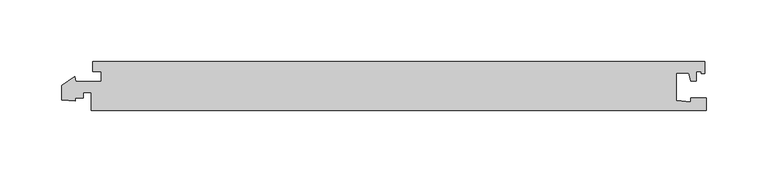
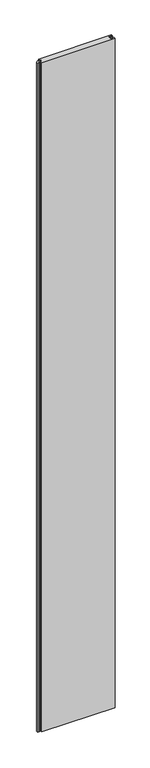
"""IFC4 building model written with IfcOpenShell, lengths in millimetres: proxy geometry, Generic Models 5:Generic Models 5:321804:Generic Models 5:321804 : Generic Models 5:Generic Models 5:321804:26 : Generic Models 5:Generic Models 5:321804:Generic Models 5:321804 : Generic Models 5:Generic Models 5:321804:300761."""

import ifcopenshell
import ifcopenshell.guid

model = None  # the IFC model being written
_history = None  # IfcOwnerHistory: only IFC2X3 demands one
_inside = {}  # id of a spatial element -> (the spatial element, [elements in it])
_under = {}  # id of a project, library or spatial element -> (it, [spatial elements below it])
_declared = {}  # id of a project -> (the project, [libraries it declares])
_typed = {}  # id of a type object -> (the type object, [elements of that type])
_made_of = {}  # id of a material, layer set ... -> (it, [elements and type objects made of it])


def new_model(schema):
    """Start an empty IFC model of exactly this schema.

    Asked for "IFC4X3", IfcOpenShell would pick the latest addendum, in which some entities
    have other attributes; the version numbers below select the first issue.
    IFC2X3 requires an IfcOwnerHistory on every rooted entity: one is made here for all.
    """
    global model, _history
    if schema == "IFC4X3":
        model = ifcopenshell.file(schema_version=(4, 3, 0, 0))
    else:
        model = ifcopenshell.file(schema=schema)
    _inside.clear()
    _under.clear()
    _declared.clear()
    _typed.clear()
    _made_of.clear()
    _history = None
    if model.schema == "IFC2X3":
        org = make("IfcOrganization", Name="unknown")
        user = make(
            "IfcPersonAndOrganization",
            ThePerson=make("IfcPerson", FamilyName="unknown"),
            TheOrganization=org,
        )
        app = make(
            "IfcApplication",
            ApplicationDeveloper=org,
            Version="unknown",
            ApplicationFullName="unknown",
            ApplicationIdentifier="unknown",
        )
        _history = make(
            "IfcOwnerHistory",
            OwningUser=user,
            OwningApplication=app,
            ChangeAction="ADDED",
            CreationDate=0,
        )
    return model


def make(cls, **values):
    """One entity of the class cls with the attributes given. An attribute that is None is left unset."""
    return model.create_entity(
        cls, **{name: value for name, value in values.items() if value is not None}
    )


def rooted(cls, **values):
    """An entity with a GlobalId (a new one), such as an element, a storey or a relation."""
    return make(cls, GlobalId=ifcopenshell.guid.new(), OwnerHistory=_history, **values)


def si_unit(unit_type, name, prefix=None):
    """IfcSIUnit, for example si_unit("LENGTHUNIT", "METRE", prefix="MILLI")."""
    return make("IfcSIUnit", UnitType=unit_type, Prefix=prefix, Name=name)


def assignment(units):
    """IfcUnitAssignment: the units of a project."""
    return None if units is None else make("IfcUnitAssignment", Units=units)


def point(xyz):
    """IfcCartesianPoint."""
    return None if xyz is None else make("IfcCartesianPoint", Coordinates=xyz)


def direction(xyz):
    """IfcDirection."""
    return None if xyz is None else make("IfcDirection", DirectionRatios=xyz)


def frame(location, z_axis=None, x_axis=None):
    """IfcAxis2Placement3D, a coordinate frame: its origin and axes. An axis left out is left unset."""
    return make(
        "IfcAxis2Placement3D",
        Location=point(location),
        Axis=direction(z_axis),
        RefDirection=direction(x_axis),
    )


def origin():
    """The frame at (0, 0, 0) with its axes left unset."""
    return frame((0.0, 0.0, 0.0))


def place(relative_to, where):
    """IfcLocalPlacement: puts the frame where relative to a parent placement (None: the world)."""
    return make(
        "IfcLocalPlacement", PlacementRelTo=relative_to, RelativePlacement=where
    )


def context(
    kind, dimensions, precision=None, world=None, true_north=None, identifier=None
):
    """IfcGeometricRepresentationContext, for example the 3D "Model" context."""
    return make(
        "IfcGeometricRepresentationContext",
        ContextIdentifier=identifier,
        ContextType=kind,
        CoordinateSpaceDimension=dimensions,
        Precision=precision,
        WorldCoordinateSystem=world,
        TrueNorth=true_north,
    )


def project(units=None, contexts=None):
    """IfcProject with its units and contexts."""
    return rooted(
        "IfcProject",
        Name="project",
        RepresentationContexts=contexts,
        UnitsInContext=assignment(units),
    )


def spatial(cls, under=None, at=None, **own):
    """A site, building, storey or space (cls), placed at a placement, below another one or the project."""
    s = rooted(cls, ObjectPlacement=at, **own)
    if under is not None:
        _under.setdefault(under.id(), (under, []))[1].append(s)
    return s


def polyline(points):
    """IfcPolyline through the points."""
    return make("IfcPolyline", Points=[point(p) for p in points])


def outline(outer, holes=None, kind="AREA"):
    """IfcArbitraryClosedProfileDef: a profile drawn as a closed curve; with holes, ...WithVoids."""
    if holes is None:
        return make("IfcArbitraryClosedProfileDef", ProfileType=kind, OuterCurve=outer)
    return make(
        "IfcArbitraryProfileDefWithVoids",
        ProfileType=kind,
        OuterCurve=outer,
        InnerCurves=holes,
    )


def extrude(swept, where, along, depth):
    """IfcExtrudedAreaSolid: the profile swept, set in the frame where, extruded along a direction by depth."""
    return make(
        "IfcExtrudedAreaSolid",
        SweptArea=swept,
        Position=where,
        ExtrudedDirection=direction(along),
        Depth=depth,
    )


def shape(context_of_items, identifier, shape_type, items):
    """IfcShapeRepresentation: the items that make up one representation, for example the "Body"."""
    return make(
        "IfcShapeRepresentation",
        ContextOfItems=context_of_items,
        RepresentationIdentifier=identifier,
        RepresentationType=shape_type,
        Items=items,
    )


def source(mapping_origin, context_of_items, identifier, shape_type, items):
    """IfcRepresentationMap: a shape defined once, which mapped items show again and again."""
    return make(
        "IfcRepresentationMap",
        MappingOrigin=mapping_origin,
        MappedRepresentation=shape(context_of_items, identifier, shape_type, items),
    )


def transform(
    local_origin,
    x_axis=None,
    y_axis=None,
    z_axis=None,
    scale=None,
    scale2=None,
    scale3=None,
    uniform=True,
):
    """IfcCartesianTransformationOperator3D, or its non-uniform kind. x_axis, y_axis, z_axis: its Axis1, 2, 3."""
    if uniform:
        return make(
            "IfcCartesianTransformationOperator3D",
            Axis1=direction(x_axis),
            Axis2=direction(y_axis),
            LocalOrigin=point(local_origin),
            Scale=scale,
            Axis3=direction(z_axis),
        )
    return make(
        "IfcCartesianTransformationOperator3DnonUniform",
        Axis1=direction(x_axis),
        Axis2=direction(y_axis),
        LocalOrigin=point(local_origin),
        Scale=scale,
        Axis3=direction(z_axis),
        Scale2=scale2,
        Scale3=scale3,
    )


def mapped(mapping_source, mapping_target):
    """IfcMappedItem: shows the shape of a source again, moved by a transform."""
    return make(
        "IfcMappedItem", MappingSource=mapping_source, MappingTarget=mapping_target
    )


def made_of(thing, what):
    """Note that an element or type object is made of a material, layer set ...; save() writes the relation."""
    if what is not None:
        _made_of.setdefault(what.id(), (what, []))[1].append(thing)
    return thing


def element(
    cls,
    number,
    at=None,
    inside=None,
    cuts=None,
    type_object=None,
    material=None,
    context=None,
    identifier="Body",
    shape_type=None,
    held_by="IfcProductDefinitionShape",
    body=None,
    shapes=None,
    **own,
):
    """One element of the class cls, such as IfcWall. Its Tag is "e" and its number.

    at: its placement. inside: the storey or other place that contains it. cuts: it is an
    opening in that element (IfcRelVoidsElement). A single representation is given by context,
    identifier, shape_type and body (its items); several are given by shapes. held_by: the class
    of the entity that holds the representations. save() writes the other relations.
    """
    e = rooted(cls, Tag="e%d" % number, ObjectPlacement=at, **own)
    if body is not None:
        shapes = [shape(context, identifier, shape_type, body)]
    if shapes is not None:
        e.Representation = make(held_by, Representations=shapes)
    if inside is not None:
        _inside.setdefault(inside.id(), (inside, []))[1].append(e)
    if cuts is not None:
        rooted(
            "IfcRelVoidsElement", RelatingBuildingElement=cuts, RelatedOpeningElement=e
        )
    if type_object is not None:
        _typed.setdefault(type_object.id(), (type_object, []))[1].append(e)
    return made_of(e, material)


def aggregate(whole, parts):
    """IfcRelAggregates: a whole, such as a stair, and the parts it consists of."""
    return rooted("IfcRelAggregates", RelatingObject=whole, RelatedObjects=parts)


def save(model, path):
    """Write the relations noted so far, then the file.

    IfcRelAggregates (storeys below a building ...), IfcRelContainedInSpatialStructure (elements
    in a storey), IfcRelDefinesByType, IfcRelAssociatesMaterial and IfcRelDeclares: one each for
    every whole, place, type object, material and project.
    """
    for whole, parts in _under.values():
        aggregate(whole, parts)
    for where, things in _inside.values():
        rooted(
            "IfcRelContainedInSpatialStructure",
            RelatedElements=things,
            RelatingStructure=where,
        )
    for kind, things in _typed.values():
        rooted("IfcRelDefinesByType", RelatedObjects=things, RelatingType=kind)
    for what, things in _made_of.values():
        rooted("IfcRelAssociatesMaterial", RelatedObjects=things, RelatingMaterial=what)
    for by, libraries in _declared.values():
        rooted("IfcRelDeclares", RelatingContext=by, RelatedDefinitions=libraries)
    model.write(path)


def generic_models_55241827(model_context):
    return source(origin(), model_context, "Body", "SweptSolid", [
        extrude(outline(polyline([(593294.8386129, -568238.0537319), (593284.4802827, -568238.0537319), (593284.4802827, -568260.5495221), (593296.4802827, -568261.5993861), (593296.4802827, -568258.3537319), (593309.2302827, -568258.3537319), (593309.2302827, -568268.5537319), (592809.2302827, -568268.5537319), (592809.2302827, -568254.0537319), (592802.6052827, -568254.0537319), (592802.6052827, -568258.3537319), (592795.9802827, -568258.3537319), (592795.9802827, -568261.0537319), (592784.9802827, -568260.0913566), (592784.9802827, -568248.2332156), (592795.6617846, -568241.1258504), (592796.7142572, -568245.0537319), (592817.4302827, -568245.0537319), (592817.4302827, -568237.0537319), (592810.4802827, -568237.0537319), (592810.4802827, -568228.5537319), (593307.9802827, -568228.5537319), (593307.9802827, -568238.5537319), (593304.9802827, -568238.5537319), (593304.9802827, -568237.0537319), (593301.0302827, -568237.0537319), (593301.0302827, -568244.5537319), (593296.5802827, -568244.5537319), (593294.8386129, -568238.0537319)])), frame((0.0, 0.0, 7716.6845784), z_axis=(0.0, 0.0, 1.0), x_axis=(1.0, 0.0, 0.0)), (0.0, 0.0, 1.0), 4819.5604755),
    ])


if __name__ == "__main__":
    model = new_model("IFC4")
    model_context = context("Model", 3, world=origin())
    ifc_project = project(units=[si_unit("LENGTHUNIT", "METRE", prefix="MILLI")], contexts=[model_context])
    site = spatial("IfcSite", under=ifc_project)
    building = spatial("IfcBuilding", under=site)
    placement = place(None, origin())
    generic_models_shape = generic_models_55241827(model_context)
    element("IfcBuildingElementProxy", 1, Name="Generic Models 5:Generic Models 5:321804:Generic Models 5:321804 : Generic Models 5:Generic Models 5:321804:26 : Generic Models 5:Generic Models 5:321804:Generic Models 5:321804 : Generic Models 5:Generic Models 5:321804:300761", ObjectType="Generic Models 5:Generic Models 5:321804:Generic Models 5:321804 : Generic Models 5:Generic Models 5:321804:26 : Generic Models 5:Generic Models 5:321804:Generic Models 5:321804 : Generic Models 5:Generic Models 5:321804:300761", at=placement, inside=building, context=model_context, shape_type="MappedRepresentation", body=[
        mapped(generic_models_shape, transform((0.0, 0.0, 0.0), x_axis=(1.0, 0.0, 0.0), y_axis=(0.0, 1.0, 0.0), z_axis=(0.0, 0.0, 1.0))),
    ])
    save(model, "model.ifc")

# Revit data of these elements
# Type "Generic Models 5:Generic Models 5:321804:Generic Models 5:321804 : Generic Models 5:Generic Models 5:321804:26 : Generic Models 5:Generic Models 5:321804:Generic Models 5:321804 : Generic Models 5:Generic Models 5:321804:300761"
#   NameOverride = "Generic Models 5:Generic Models 5:321804:Generic Models 5:321804 : Generic Models 5:Generic Models 5:321804:300761"
#   ObjectTypeOverride = "Generic Models 5:321804 : Generic Models 5:Generic Models 5:321804"
#   Reference = "Generic Models 5"
#   Tag = "300761"
# Element 1 (IfcBuildingElementProxy, "Generic Models 5:Generic Models 5:321804:Generic Models 5:321804 : Generic Models 5:Generic Models 5:321804:26 : Generic Models 5:Generic Models 5:321804:Generic Models 5:321804 : Generic Models 5:Generic Models 5:321804:300761")
#   Materials on its faces: "POLYCARBONATE PANEL - ARCOPLUS 547"
# Materials
#   "POLYCARBONATE PANEL - ARCOPLUS 547": class "Unassigned", colour RGB 202 225 249, transparency 0.45, Cost = 0
